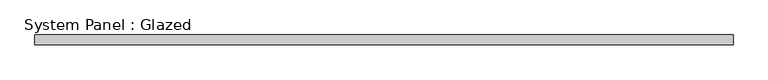
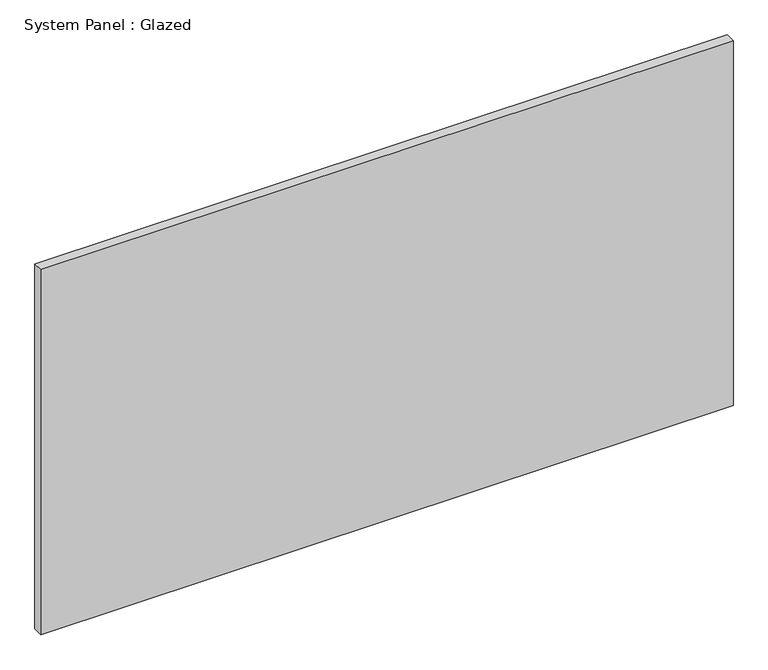
"""IFC4 building model written with IfcOpenShell, lengths in millimetres: plate geometry, System Panel : Glazed."""

from ifc_helpers import new_model, si_unit, origin, origin_with_axes, place, context, project, spatial, polyline, outline, extrude, source, transform, mapped, element, save


def system_panel_glazed_9c29bfcc(model_context):
    return source(origin(), model_context, "Body", "SweptSolid", [
        extrude(outline(polyline([(874.2727273, 24.5), (-874.2727273, 24.5), (-874.2727273, 49.5), (874.2727273, 49.5), (874.2727273, 24.5)])), origin_with_axes(), (0.0, 0.0, 1.0), 975.0),
    ])


if __name__ == "__main__":
    model = new_model("IFC4")
    model_context = context("Model", 3, world=origin())
    ifc_project = project(units=[si_unit("LENGTHUNIT", "METRE", prefix="MILLI")], contexts=[model_context])
    site = spatial("IfcSite", under=ifc_project)
    building = spatial("IfcBuilding", under=site)
    placement = place(None, origin())
    system_panel_glazed_shape = system_panel_glazed_9c29bfcc(model_context)
    element("IfcPlate", 1, ObjectType="System Panel : Glazed", at=placement, inside=building, context=model_context, shape_type="MappedRepresentation", body=[
        mapped(system_panel_glazed_shape, transform((0.0, 0.0, 0.0), x_axis=(1.0, 0.0, 0.0), y_axis=(0.0, 1.0, 0.0), z_axis=(0.0, 0.0, 1.0))),
    ])
    save(model, "model.ifc")

# Revit data of these elements
# Element 1 (IfcPlate, "System Panel : Glazed")
#   Materials on its faces: "Glass"
# Materials
#   "Glass": class "Glass", colour RGB 218 227 224, transparency 0.85, Description = "Soda Lime Glass", Cost = 0
